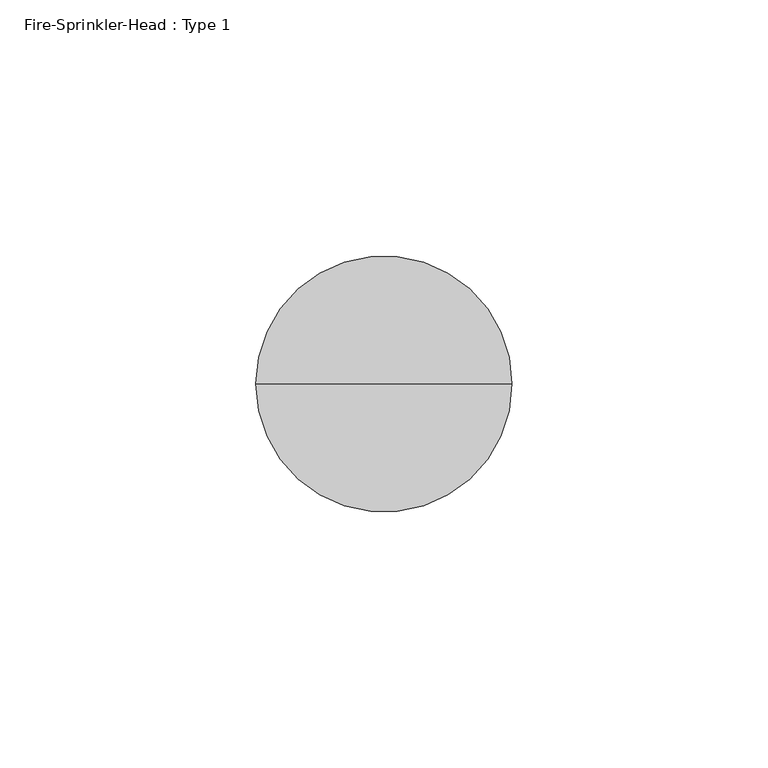
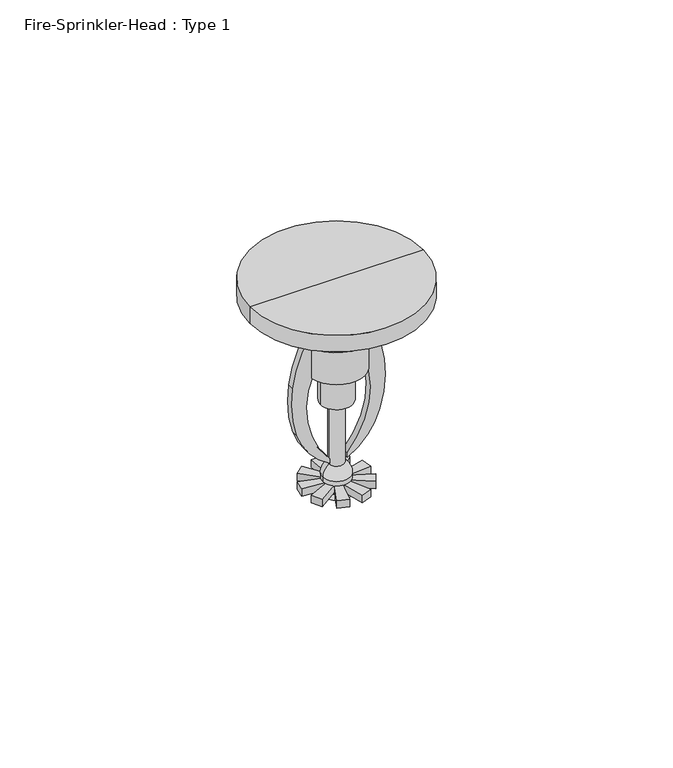
"""IFC4 building model written with IfcOpenShell, lengths in millimetres: alarm geometry, Fire-Sprinkler-Head : Type 1."""

from ifc_helpers import new_model, si_unit, point, frame, frame_2d, origin, place, context, project, spatial, polyline, circle_curve, ellipse_curve, trimmed, segment, composite_curve, outline, extrude, source, transform, mapped, element, save
from ifc_brep_helpers import plane_surface, cylinder_surface, revolved_surface, advanced_brep


def fire_sprinkler_head_type_1_89d12226(model_context):
    return source(origin(), model_context, "Body", "SolidModel", [
        extrude(outline(composite_curve([segment(polyline([(3978.349287, 0.0), (3978.349287, 4.8492465)]), True, "CONTINUOUS"), segment(trimmed(circle_curve(frame_2d((3963.8626562, -16.7101966)), 25.9744501), [point((3978.349287, 4.8492465))], [point((3946.4410747, 2.555331))], True, "CARTESIAN"), True, "CONTINUOUS"), segment(polyline([(3946.4410747, 2.555331), (3945.0501011, 2.555331)]), True, "CONTINUOUS"), segment(trimmed(circle_curve(frame_2d((3962.5874819, -7.1839127)), 20.0602242), [point((3945.0501011, 2.555331))], [point((3956.7072905, 11.9951369))], False, "CARTESIAN"), True, "CONTINUOUS"), segment(trimmed(circle_curve(frame_2d((3966.9398015, -21.3795994)), 34.9081266), [point((3956.7072905, 11.9951369))], [point((3971.4511948, 13.2357821))], False, "CARTESIAN"), True, "CONTINUOUS"), segment(trimmed(circle_curve(frame_2d((3966.6562283, -22.8835825)), 36.4362484), [point((3971.4511948, 13.2357821))], [point((3985.8319856, 8.0985177))], False, "CARTESIAN"), True, "CONTINUOUS"), segment(polyline([(3985.8319856, 8.0985177), (3985.8319856, 0.0), (3978.349287, 0.0)]), True, "CONTINUOUS")], self_intersect=False)), frame((0.0, -0.987392, 0.0), z_axis=(0.0, 1.0, 0.0), x_axis=(0.0, 0.0, 1.0)), (0.0, 0.0, 1.0), 2.0345161),
        extrude(outline(polyline([(9.9808686, 0.1084998), (0.132791, -0.7530953), (-0.132791, 0.7530953), (9.4160577, 3.3117016), (9.9808686, 0.1084998)])), frame((0.0, 0.0, 3936.8211831), z_axis=(0.0, 0.0, 1.0), x_axis=(1.0, 0.0, 0.0)), (0.0, 0.0, 1.0), 2.2906652),
        extrude(outline(polyline([(7.7155312, -6.332463), (-0.3823565, -0.6622609), (0.3823565, 0.6622609), (9.3418394, -3.5156146), (7.7155312, -6.332463)])), frame((0.0, 0.0, 3936.8211831), z_axis=(0.0, 0.0, 1.0), x_axis=(1.0, 0.0, 0.0)), (0.0, 0.0, 1.0), 2.2906652),
        extrude(outline(polyline([(1.8400111, -9.8103959), (-0.7185952, -0.2615473), (0.7185952, 0.2615473), (4.8964707, -8.6979356), (1.8400111, -9.8103959)])), frame((0.0, 0.0, 3936.8211831), z_axis=(0.0, 0.0, 1.0), x_axis=(1.0, 0.0, 0.0)), (0.0, 0.0, 1.0), 2.2906652),
        extrude(outline(polyline([(-4.8964707, -8.6979356), (-0.7185952, 0.2615473), (0.7185952, -0.2615473), (-1.8400111, -9.8103959), (-4.8964707, -8.6979356)])), frame((0.0, 0.0, 3936.8211831), z_axis=(0.0, 0.0, 1.0), x_axis=(1.0, 0.0, 0.0)), (0.0, 0.0, 1.0), 2.2906652),
        extrude(outline(polyline([(-9.3418394, -3.5156146), (-0.3823565, 0.6622609), (0.3823565, -0.6622609), (-7.7155312, -6.332463), (-9.3418394, -3.5156146)])), frame((0.0, 0.0, 3936.8211831), z_axis=(0.0, 0.0, 1.0), x_axis=(1.0, 0.0, 0.0)), (0.0, 0.0, 1.0), 2.2906652),
        extrude(outline(polyline([(-9.4160577, 3.3117016), (0.132791, 0.7530953), (-0.132791, -0.7530953), (-9.9808686, 0.1084998), (-9.4160577, 3.3117016)])), frame((0.0, 0.0, 3936.8211831), z_axis=(0.0, 0.0, 1.0), x_axis=(1.0, 0.0, 0.0)), (0.0, 0.0, 1.0), 2.2906652),
        extrude(outline(polyline([(-5.0843979, 8.5894358), (0.5858042, 0.4915481), (-0.5858042, -0.4915481), (-7.5760466, 6.4986943), (-5.0843979, 8.5894358)])), frame((0.0, 0.0, 3936.8211831), z_axis=(0.0, 0.0, 1.0), x_axis=(1.0, 0.0, 0.0)), (0.0, 0.0, 1.0), 2.2906652),
        extrude(outline(polyline([(7.5760466, 6.4986943), (0.5858042, -0.4915481), (-0.5858042, 0.4915481), (5.0843979, 8.5894358), (7.5760466, 6.4986943)])), frame((0.0, 0.0, 3936.8211831), z_axis=(0.0, 0.0, 1.0), x_axis=(1.0, 0.0, 0.0)), (0.0, 0.0, 1.0), 2.2906652),
        extrude(outline(polyline([(1.6263082, 9.8480775), (0.764713, 0.0), (-0.764713, 0.0), (-1.6263082, 9.8480775), (1.6263082, 9.8480775)])), frame((0.0, 0.0, 3936.8211831), z_axis=(0.0, 0.0, 1.0), x_axis=(1.0, 0.0, 0.0)), (0.0, 0.0, 1.0), 2.2906652),
        extrude(outline(composite_curve([segment(polyline([(3978.349287, 0.0), (3985.8319856, 0.0), (3985.8319856, -8.0985177)]), True, "CONTINUOUS"), segment(trimmed(circle_curve(frame_2d((3966.6562283, 22.8835825)), 36.4362484), [point((3985.8319856, -8.0985177))], [point((3971.4511948, -13.2357821))], False, "CARTESIAN"), True, "CONTINUOUS"), segment(trimmed(circle_curve(frame_2d((3966.9398015, 21.3795994)), 34.9081266), [point((3971.4511948, -13.2357821))], [point((3956.7072905, -11.9951369))], False, "CARTESIAN"), True, "CONTINUOUS"), segment(trimmed(circle_curve(frame_2d((3962.5874819, 7.1839127)), 20.0602242), [point((3956.7072905, -11.9951369))], [point((3945.0501011, -2.555331))], False, "CARTESIAN"), True, "CONTINUOUS"), segment(polyline([(3945.0501011, -2.555331), (3946.4410747, -2.555331)]), True, "CONTINUOUS"), segment(trimmed(circle_curve(frame_2d((3963.8626562, 16.7101966)), 25.9744501), [point((3946.4410747, -2.555331))], [point((3978.349287, -4.8492465))], True, "CARTESIAN"), True, "CONTINUOUS"), segment(polyline([(3978.349287, -4.8492465), (3978.349287, 0.0)]), True, "CONTINUOUS")], self_intersect=False)), frame((0.0, -0.987392, 0.0), z_axis=(0.0, 1.0, 0.0), x_axis=(0.0, 0.0, 1.0)), (0.0, 0.0, 1.0), 2.0345161),
        advanced_brep(
        [(25.0, 0.0, 3995.0), (-25.0, 0.0, 3995.0), (-25.0, 0.0, 4000.0), (25.0, 0.0, 4000.0), (18.8042198, 0.0, 3995.0), (-18.8042198, 0.0, 3995.0), (12.2416631, 0.0, 3991.6324601), (-12.2416631, 0.0, 3991.6324601), (12.2416631, 0.0, 3985.8319856), (-12.2416631, 0.0, 3985.8319856), (8.0985177, 0.0, 3985.8319856), (-8.0985177, 0.0, 3985.8319856), (8.0985177, 0.0, 3973.1223694), (-8.0985177, 0.0, 3973.1223694), (4.6513455, 0.0, 3973.1223694), (-4.6513455, 0.0, 3973.1223694), (4.6513455, 0.0, 3963.1223694), (-4.6513455, 0.0, 3963.1223694), (2.1931757, 0.0, 3963.1223694), (-2.1931757, 0.0, 3963.1223694), (2.1931757, 0.0, 3944.1533344), (-2.1931757, 0.0, 3944.1533344), (4.0228103, 0.0, 3940.7527841), (-4.0228103, 0.0, 3940.7527841), (4.0228103, 0.0, 3939.1118483), (-4.0228103, 0.0, 3939.1118483), (1.2979197, 0.0, 3939.1118483), (-1.2979197, 0.0, 3939.1118483), (1.2979197, 0.0, 3936.9618068), (-1.2979197, 0.0, 3936.9618068), (4.3349972, 0.0, 3936.9618068), (-4.3349972, 0.0, 3936.9618068), (4.3349972, 0.0, 3935.4284458), (-4.3349972, 0.0, 3935.4284458), (0.0, 0.0, 3935.4284458), (0.0, 0.0, 4000.0)],
        [
            (0, 1, circle_curve(frame((0.0, 0.0, 3995.0), z_axis=(0.0, 0.0, 1.0), x_axis=(-1.0, 0.0, 0.0)), 25.0)),
            (1, 2),
            (2, 3, circle_curve(frame((0.0, 0.0, 4000.0), z_axis=(0.0, 0.0, -1.0), x_axis=(-1.0, 0.0, 0.0)), 25.0)),
            (3, 0),
            (1, 0, circle_curve(frame((0.0, 0.0, 3995.0), z_axis=(0.0, 0.0, 1.0), x_axis=(-1.0, 0.0, 0.0)), 25.0)),
            (3, 2, circle_curve(frame((0.0, 0.0, 4000.0), z_axis=(0.0, 0.0, -1.0), x_axis=(-1.0, 0.0, 0.0)), 25.0)),
            (4, 5, circle_curve(frame((0.0, 0.0, 3995.0), z_axis=(0.0, 0.0, 1.0), x_axis=(-1.0, 0.0, 0.0)), 18.8042198)),
            (5, 1),
            (0, 4),
            (5, 4, circle_curve(frame((0.0, 0.0, 3995.0), z_axis=(0.0, 0.0, 1.0), x_axis=(-1.0, 0.0, 0.0)), 18.8042198)),
            (6, 7, circle_curve(frame((0.0, 0.0, 3991.6324601), z_axis=(0.0, 0.0, 1.0), x_axis=(-1.0, 0.0, 0.0)), 12.2416631)),
            (7, 5, circle_curve(frame((-4.8124083, 0.0, 4014.1885825), z_axis=(0.0, 1.0, 0.0), x_axis=(-1.0, 0.0, 0.0)), 23.7481049)),
            (4, 6, circle_curve(frame((4.8124083, 0.0, 4014.1885825), z_axis=(0.0, 1.0, 0.0), x_axis=(1.0, 0.0, 0.0)), 23.7481049)),
            (7, 6, circle_curve(frame((0.0, 0.0, 3991.6324601), z_axis=(0.0, 0.0, 1.0), x_axis=(-1.0, 0.0, 0.0)), 12.2416631)),
            (8, 9, circle_curve(frame((0.0, 0.0, 3985.8319856), z_axis=(0.0, 0.0, 1.0), x_axis=(-1.0, 0.0, 0.0)), 12.2416631)),
            (9, 7),
            (6, 8),
            (9, 8, circle_curve(frame((0.0, 0.0, 3985.8319856), z_axis=(0.0, 0.0, 1.0), x_axis=(-1.0, 0.0, 0.0)), 12.2416631)),
            (10, 11, circle_curve(frame((0.0, 0.0, 3985.8319856), z_axis=(0.0, 0.0, 1.0), x_axis=(-1.0, 0.0, 0.0)), 8.0985177)),
            (11, 9),
            (8, 10),
            (11, 10, circle_curve(frame((0.0, 0.0, 3985.8319856), z_axis=(0.0, 0.0, 1.0), x_axis=(-1.0, 0.0, 0.0)), 8.0985177)),
            (12, 13, circle_curve(frame((0.0, 0.0, 3973.1223694), z_axis=(0.0, 0.0, 1.0), x_axis=(-1.0, 0.0, 0.0)), 8.0985177)),
            (13, 11),
            (10, 12),
            (13, 12, circle_curve(frame((0.0, 0.0, 3973.1223694), z_axis=(0.0, 0.0, 1.0), x_axis=(-1.0, 0.0, 0.0)), 8.0985177)),
            (14, 15, circle_curve(frame((0.0, 0.0, 3973.1223694), z_axis=(0.0, 0.0, 1.0), x_axis=(-1.0, 0.0, 0.0)), 4.6513455)),
            (15, 13),
            (12, 14),
            (15, 14, circle_curve(frame((0.0, 0.0, 3973.1223694), z_axis=(0.0, 0.0, 1.0), x_axis=(-1.0, 0.0, 0.0)), 4.6513455)),
            (16, 17, circle_curve(frame((0.0, 0.0, 3963.1223694), z_axis=(0.0, 0.0, 1.0), x_axis=(-1.0, 0.0, 0.0)), 4.6513455)),
            (17, 15),
            (14, 16),
            (17, 16, circle_curve(frame((0.0, 0.0, 3963.1223694), z_axis=(0.0, 0.0, 1.0), x_axis=(-1.0, 0.0, 0.0)), 4.6513455)),
            (18, 19, circle_curve(frame((0.0, 0.0, 3963.1223694), z_axis=(0.0, 0.0, 1.0), x_axis=(-1.0, 0.0, 0.0)), 2.1931757)),
            (19, 17),
            (16, 18),
            (19, 18, circle_curve(frame((0.0, 0.0, 3963.1223694), z_axis=(0.0, 0.0, 1.0), x_axis=(-1.0, 0.0, 0.0)), 2.1931757)),
            (20, 21, circle_curve(frame((0.0, 0.0, 3944.1533344), z_axis=(0.0, 0.0, 1.0), x_axis=(-1.0, 0.0, 0.0)), 2.1931757)),
            (21, 19),
            (18, 20),
            (21, 20, circle_curve(frame((0.0, 0.0, 3944.1533344), z_axis=(0.0, 0.0, 1.0), x_axis=(-1.0, 0.0, 0.0)), 2.1931757)),
            (22, 23, circle_curve(frame((0.0, 0.0, 3940.7527841), z_axis=(0.0, 0.0, 1.0), x_axis=(-1.0, 0.0, 0.0)), 4.0228103)),
            (23, 21, circle_curve(frame((0.3386488, 0.0, 3940.5986256), z_axis=(0.0, 1.0, 0.0), x_axis=(-1.0, 0.0, 0.0)), 4.3641826)),
            (20, 22, circle_curve(frame((-0.3386488, 0.0, 3940.5986256), z_axis=(0.0, 1.0, 0.0), x_axis=(1.0, 0.0, 0.0)), 4.3641826)),
            (23, 22, circle_curve(frame((0.0, 0.0, 3940.7527841), z_axis=(0.0, 0.0, 1.0), x_axis=(-1.0, 0.0, 0.0)), 4.0228103)),
            (24, 25, circle_curve(frame((0.0, 0.0, 3939.1118483), z_axis=(0.0, 0.0, 1.0), x_axis=(-1.0, 0.0, 0.0)), 4.0228103)),
            (25, 23),
            (22, 24),
            (25, 24, circle_curve(frame((0.0, 0.0, 3939.1118483), z_axis=(0.0, 0.0, 1.0), x_axis=(-1.0, 0.0, 0.0)), 4.0228103)),
            (26, 27, circle_curve(frame((0.0, 0.0, 3939.1118483), z_axis=(0.0, 0.0, 1.0), x_axis=(-1.0, 0.0, 0.0)), 1.2979197)),
            (27, 25),
            (24, 26),
            (27, 26, circle_curve(frame((0.0, 0.0, 3939.1118483), z_axis=(0.0, 0.0, 1.0), x_axis=(-1.0, 0.0, 0.0)), 1.2979197)),
            (28, 29, circle_curve(frame((0.0, 0.0, 3936.9618068), z_axis=(0.0, 0.0, 1.0), x_axis=(-1.0, 0.0, 0.0)), 1.2979197)),
            (29, 27),
            (26, 28),
            (29, 28, circle_curve(frame((0.0, 0.0, 3936.9618068), z_axis=(0.0, 0.0, 1.0), x_axis=(-1.0, 0.0, 0.0)), 1.2979197)),
            (30, 31, circle_curve(frame((0.0, 0.0, 3936.9618068), z_axis=(0.0, 0.0, 1.0), x_axis=(-1.0, 0.0, 0.0)), 4.3349972)),
            (31, 29),
            (28, 30),
            (31, 30, circle_curve(frame((0.0, 0.0, 3936.9618068), z_axis=(0.0, 0.0, 1.0), x_axis=(-1.0, 0.0, 0.0)), 4.3349972)),
            (32, 33, circle_curve(frame((0.0, 0.0, 3935.4284458), z_axis=(0.0, 0.0, 1.0), x_axis=(-1.0, 0.0, 0.0)), 4.3349972)),
            (33, 31, circle_curve(frame((-4.3349972, 0.0, 3936.1951263), z_axis=(0.0, 1.0, 0.0), x_axis=(-1.0, 0.0, 0.0)), 0.7666805)),
            (30, 32, circle_curve(frame((4.3349972, 0.0, 3936.1951263), z_axis=(0.0, 1.0, 0.0), x_axis=(1.0, 0.0, 0.0)), 0.7666805)),
            (33, 32, circle_curve(frame((0.0, 0.0, 3935.4284458), z_axis=(0.0, 0.0, 1.0), x_axis=(-1.0, 0.0, 0.0)), 4.3349972)),
            (34, 33),
            (32, 34),
            (2, 35),
            (35, 3),
        ],
        [
            cylinder_surface(frame((0.0, 0.0, 3925.1994284), z_axis=(0.0, 0.0, -1.0), x_axis=(-1.0, 0.0, 0.0)), 25.0),
            plane_surface(frame((0.0, 0.0, 3995.0), z_axis=(0.0, 0.0, -1.0), x_axis=(-1.0, 0.0, 0.0))),
            revolved_surface(trimmed(ellipse_curve(frame((-4.8124083, 0.0, 4014.1885825), z_axis=(0.0, -1.0, 0.0), x_axis=(-1.0, 0.0, 0.0)), 23.7481049, 23.7481049), [point((-18.8042198, 0.0, 3995.0))], [point((-12.2416631, 0.0, 3991.6324601))], True, "CARTESIAN"), (0.0, 0.0, 3925.1994284), (0.0, 0.0, -1.0)),
            cylinder_surface(frame((0.0, 0.0, 3925.1994284), z_axis=(0.0, 0.0, -1.0), x_axis=(-1.0, 0.0, 0.0)), 12.2416631),
            plane_surface(frame((0.0, 0.0, 3985.8319856), z_axis=(0.0, 0.0, -1.0), x_axis=(-1.0, 0.0, 0.0))),
            cylinder_surface(frame((0.0, 0.0, 3925.1994284), z_axis=(0.0, 0.0, -1.0), x_axis=(-1.0, 0.0, 0.0)), 8.0985177),
            plane_surface(frame((0.0, 0.0, 3973.1223694), z_axis=(0.0, 0.0, -1.0), x_axis=(-1.0, 0.0, 0.0))),
            cylinder_surface(frame((0.0, 0.0, 3925.1994284), z_axis=(0.0, 0.0, -1.0), x_axis=(-1.0, 0.0, 0.0)), 4.6513455),
            plane_surface(frame((0.0, 0.0, 3963.1223694), z_axis=(0.0, 0.0, -1.0), x_axis=(-1.0, 0.0, 0.0))),
            cylinder_surface(frame((0.0, 0.0, 3925.1994284), z_axis=(0.0, 0.0, -1.0), x_axis=(-1.0, 0.0, 0.0)), 2.1931757),
            revolved_surface(trimmed(ellipse_curve(frame((0.3386488, 0.0, 3940.5986256), z_axis=(0.0, -1.0, 0.0), x_axis=(-1.0, 0.0, 0.0)), 4.3641826, 4.3641826), [point((-2.1931757, 0.0, 3944.1533344))], [point((-4.0228103, 0.0, 3940.7527841))], True, "CARTESIAN"), (0.0, 0.0, 3925.1994284), (0.0, 0.0, -1.0)),
            cylinder_surface(frame((0.0, 0.0, 3925.1994284), z_axis=(0.0, 0.0, -1.0), x_axis=(-1.0, 0.0, 0.0)), 4.0228103),
            plane_surface(frame((0.0, 0.0, 3939.1118483), z_axis=(0.0, 0.0, -1.0), x_axis=(-1.0, 0.0, 0.0))),
            cylinder_surface(frame((0.0, 0.0, 3925.1994284), z_axis=(0.0, 0.0, -1.0), x_axis=(-1.0, 0.0, 0.0)), 1.2979197),
            plane_surface(frame((0.0, 0.0, 3936.9618068), z_axis=(0.0, 0.0, 1.0), x_axis=(-1.0, 0.0, 0.0))),
            revolved_surface(trimmed(ellipse_curve(frame((-4.3349972, 0.0, 3936.1951263), z_axis=(0.0, -1.0, 0.0), x_axis=(-1.0, 0.0, 0.0)), 0.7666805, 0.7666805), [point((-4.3349972, 0.0, 3936.9618068))], [point((-4.3349972, 0.0, 3935.4284458))], True, "CARTESIAN"), (0.0, 0.0, 3925.1994284), (0.0, 0.0, -1.0)),
            plane_surface(frame((0.0, 0.0, 3935.4284458), z_axis=(0.0, 0.0, -1.0), x_axis=(-1.0, 0.0, 0.0))),
            plane_surface(frame((0.0, 0.0, 4000.0), z_axis=(0.0, 0.0, 1.0), x_axis=(-1.0, 0.0, 0.0))),
        ],
        [
            (0, [[1, 2, 3, 4]]),
            (0, [[5, -4, 6, -2]]),
            (1, [[7, 8, -1, 9]]),
            (1, [[10, -9, -5, -8]]),
            (2, [[11, 12, -7, 13]]),
            (2, [[14, -13, -10, -12]]),
            (3, [[15, 16, -11, 17]]),
            (3, [[18, -17, -14, -16]]),
            (4, [[19, 20, -15, 21]]),
            (4, [[22, -21, -18, -20]]),
            (5, [[23, 24, -19, 25]]),
            (5, [[26, -25, -22, -24]]),
            (6, [[27, 28, -23, 29]]),
            (6, [[30, -29, -26, -28]]),
            (7, [[31, 32, -27, 33]]),
            (7, [[34, -33, -30, -32]]),
            (8, [[35, 36, -31, 37]]),
            (8, [[38, -37, -34, -36]]),
            (9, [[39, 40, -35, 41]]),
            (9, [[42, -41, -38, -40]]),
            (10, [[43, 44, -39, 45]]),
            (10, [[46, -45, -42, -44]]),
            (11, [[47, 48, -43, 49]]),
            (11, [[50, -49, -46, -48]]),
            (12, [[51, 52, -47, 53]]),
            (12, [[54, -53, -50, -52]]),
            (13, [[55, 56, -51, 57]]),
            (13, [[58, -57, -54, -56]]),
            (14, [[59, 60, -55, 61]]),
            (14, [[62, -61, -58, -60]]),
            (15, [[63, 64, -59, 65]]),
            (15, [[66, -65, -62, -64]]),
            (16, [[67, -63, 68]]),
            (16, [[-68, -66, -67]]),
            (17, [[-3, 69, 70]]),
            (17, [[-6, -70, -69]]),
        ],
    ),
    ])


if __name__ == "__main__":
    model = new_model("IFC4")
    model_context = context("Model", 3, world=origin())
    ifc_project = project(units=[si_unit("LENGTHUNIT", "METRE", prefix="MILLI")], contexts=[model_context])
    site = spatial("IfcSite", under=ifc_project)
    building = spatial("IfcBuilding", under=site)
    placement = place(None, origin())
    fire_sprinkler_head_type_1_shape = fire_sprinkler_head_type_1_89d12226(model_context)
    element("IfcAlarm", 1, ObjectType="Fire-Sprinkler-Head : Type 1", at=placement, inside=building, context=model_context, shape_type="MappedRepresentation", body=[
        mapped(fire_sprinkler_head_type_1_shape, transform((0.0, 0.0, 0.0), x_axis=(1.0, 0.0, 0.0), y_axis=(0.0, 1.0, 0.0), z_axis=(0.0, 0.0, 1.0))),
    ])
    save(model, "model.ifc")

# Revit data of these elements
# Type "Fire-Sprinkler-Head : Type 1"
#   URL = "http://www.arcat.com/"
#   Test Data = ""
#   Temp Range = "50F / 100F over Ambient"
#   Specification = "http://www.arcat.com/divs/sec/sec13930.shtml"
#   Sales Information = ""
#   Product Properties = "http://www.arcat.com/bim/bim_info.pl?fn=Fire-Sprinkler-Head"
#   Product Data = "http://www.arcat.com/divs/sec/sec13930.shtml"
#   Model = "Generic"
#   Manufacturer Website = "http://www.arcat.com/"
#   Manufacturer Phone - Toll Free = ""
#   Manufacturer Phone = "(203) 929-9444"
#   Manufacturer Fax = "(203) 929-9444"
#   Manufacturer Email = "bim@arcat.com"
#   Manufacturer Address = "1077 Bridgeport Ave, Shelton, CT  06484"
#   Manufacturer = "Generic"
#   Keynote = "13930"
#   Installation_Fabrication = ""
#   Installation Phase = ""
#   Green Building - LEED = "http://www.arcat.com/green/green_building.shtml"
#   Drawn By = "Robert S. Weygant. CSI, CDT, SCIP"
#   Description = "17/32 Sprinkler Head"
#   Copyright = "2008, ARCAT, Inc."
#   Construction Details = "http://www.arcat.com/divs/sec/sec13930.shtml"
#   Connection Type = "1/2\" Threaded"
#   Building Codes = ""
#   Assembly Code = "D4030"
#   Sprinkler Density_GPM/Ft2 = 0.15
#   Orifice Size = 0' - 0 17/32"
#   Max Area / Sprinkler = 300 SF
#   Max Area / Riser = 52000 SF
#   Warranty Duration (Years) = 1
#   UL Listed = yes
#   Operating Pressure_Psi = 50
#   NFPA 13 Compliant = yes
#   Min Pressure_Psi = 7
#   Maintenance Schedule (Months) = 6
#   Hose Allowance_GPM = 500
#   FM Listed = yes
#   Expected Lifespan (Years) = 10
#   Tip Material = FRY REGLET REVEAL
#   Body Material = EXISTING SPRINKLER HEADS TO REMAIN
# Element 1 (IfcAlarm, "Fire-Sprinkler-Head : Type 1")
#   Materials on its faces: "EXISTING SPRINKLER HEADS TO REMAIN", "FRY REGLET REVEAL"
# Materials
#   "FRY REGLET REVEAL": class "Unassigned", colour RGB 246 240 166, transparency 0, Cost = 0
#   "EXISTING SPRINKLER HEADS TO REMAIN": class "Unassigned", colour RGB 247 247 247, transparency 0, Cost = 0
